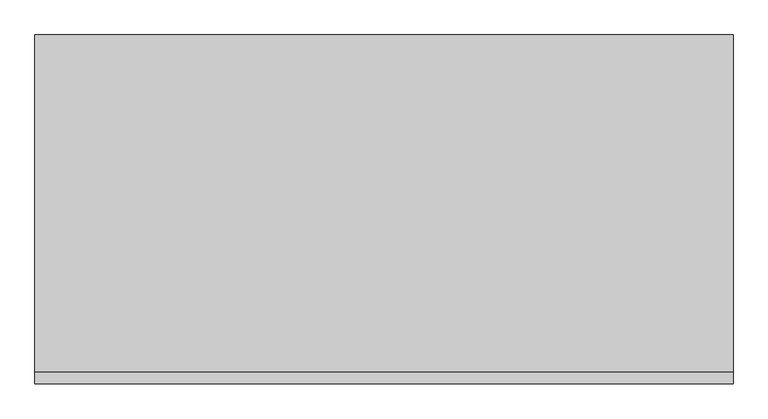
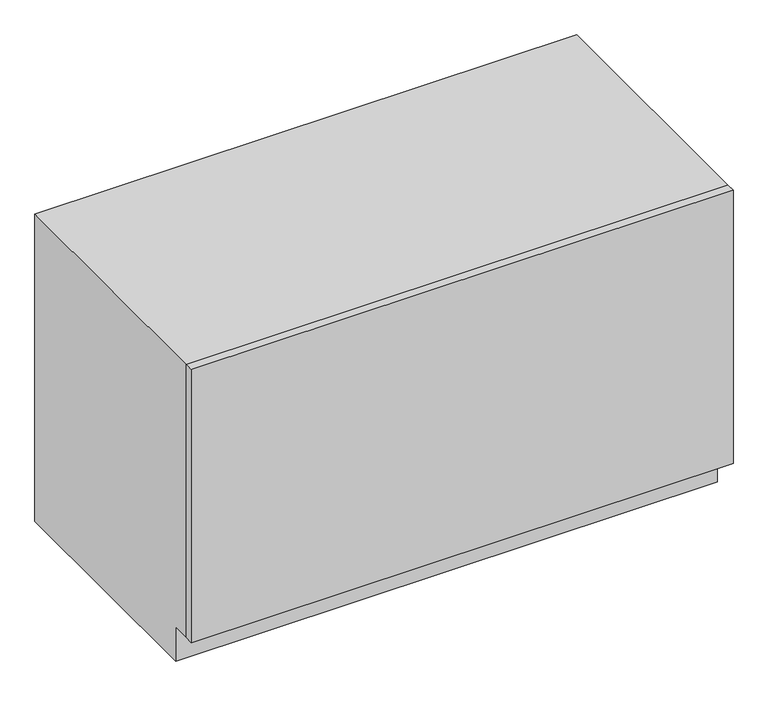
"""IFC4 building model written with IfcOpenShell, lengths in millimetres: furniture geometry, OD_CW_Base Cabinet : OD_CW_Base Cabinet."""

from ifc_helpers import new_model, si_unit, frame, origin, place, context, project, spatial, polyline, outline, extrude, source, transform, mapped, element, save


def furniture_d03e2d84(model_context):
    return source(origin(), model_context, "Body", "SweptSolid", [
        extrude(outline(polyline([(18.7377049, -127.0), (1542.7377049, -127.0), (1542.7377049, -152.4), (18.7377049, -152.4), (18.7377049, -127.0)])), frame((0.0, 0.0, 101.6), z_axis=(0.0, 0.0, 1.0), x_axis=(1.0, 0.0, 0.0)), (0.0, 0.0, 1.0), 812.8),
        extrude(outline(polyline([(-127.0, 914.4), (609.6, 914.4), (609.6, 0.0), (-76.2, 0.0), (-76.2, 101.6), (-127.0, 101.6), (-127.0, 914.4)])), frame((18.7377049, 0.0, 0.0), z_axis=(1.0, 0.0, 0.0), x_axis=(0.0, 1.0, 0.0)), (0.0, 0.0, 1.0), 1524.0),
    ])


if __name__ == "__main__":
    model = new_model("IFC4")
    model_context = context("Model", 3, world=origin())
    ifc_project = project(units=[si_unit("LENGTHUNIT", "METRE", prefix="MILLI")], contexts=[model_context])
    site = spatial("IfcSite", under=ifc_project)
    building = spatial("IfcBuilding", under=site)
    placement = place(None, origin())
    furniture_shape = furniture_d03e2d84(model_context)
    element("IfcFurniture", 1, ObjectType="OD_CW_Base Cabinet : OD_CW_Base Cabinet", at=placement, inside=building, context=model_context, shape_type="MappedRepresentation", body=[
        mapped(furniture_shape, transform((0.0, 0.0, 0.0), x_axis=(1.0, 0.0, 0.0), y_axis=(0.0, 1.0, 0.0), z_axis=(0.0, 0.0, 1.0))),
    ])
    save(model, "model.ifc")

# Revit data of these elements
# Type "OD_CW_Base Cabinet : OD_CW_Base Cabinet"
#   OD_CW_Width [instance default] = 2' - 10"
#   OD_CW_Length [instance default] = 8' - 0"
#   OD_CW_Height [instance default] = 2' - 3"
#   Depth = 2' - 0"
#   Height = 3' - 0"
#   Width = 4' - 0"
#   OD_CW_Material_Front Panel [instance default] = none
#   OD_CW_Material_Body [instance default] = none
# Element 1 (IfcFurniture, "OD_CW_Base Cabinet : OD_CW_Base Cabinet")
#   OD_CW_Width = 2' - 6"
#   OD_CW_Length = 5' - 0"
#   OD_CW_Height = 3' - 0"
#   OD_CW_Material_Body = PREP TABLE
#   Materials on its faces: "PREP TABLE", "CASEWORK"
# Materials
#   "PREP TABLE": class "Generic", colour RGB 187 187 187, transparency 0, Cost = 0
#   "CASEWORK": class "Generic", colour RGB 181 181 181, transparency 0, Cost = 0
